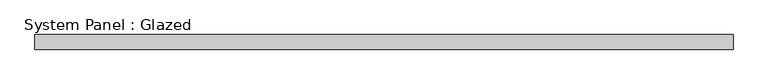
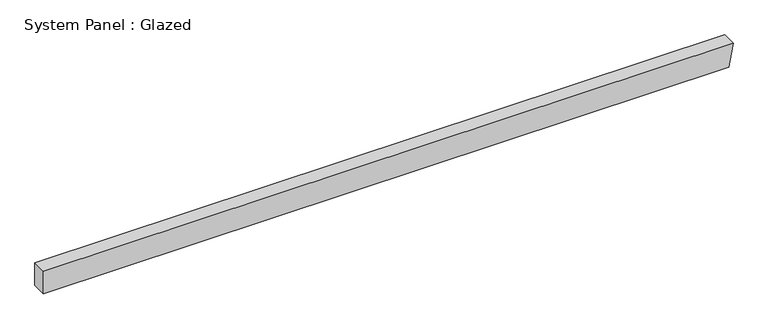
"""IFC4 building model written with IfcOpenShell, lengths in millimetres: plate geometry, System Panel : Glazed."""

from ifc_helpers import new_model, si_unit, frame, origin, place, context, project, spatial, polyline, outline, extrude, source, transform, mapped, element, save


def system_panel_glazed_abe217f1(model_context):
    return source(origin(), model_context, "Body", "SweptSolid", [
        extrude(outline(polyline([(0.0, -605.3523878), (0.0, 597.989887), (41.9143134, 605.3523878), (41.9143134, -605.3523878), (0.0, -605.3523878)])), frame((0.0, -44.45, 0.0), z_axis=(0.0, 1.0, 0.0), x_axis=(0.0, 0.0, 1.0)), (0.0, 0.0, 1.0), 25.4),
    ])


if __name__ == "__main__":
    model = new_model("IFC4")
    model_context = context("Model", 3, world=origin())
    ifc_project = project(units=[si_unit("LENGTHUNIT", "METRE", prefix="MILLI")], contexts=[model_context])
    site = spatial("IfcSite", under=ifc_project)
    building = spatial("IfcBuilding", under=site)
    placement = place(None, origin())
    system_panel_glazed_shape = system_panel_glazed_abe217f1(model_context)
    element("IfcPlate", 1, ObjectType="System Panel : Glazed", at=placement, inside=building, context=model_context, shape_type="MappedRepresentation", body=[
        mapped(system_panel_glazed_shape, transform((0.0, 0.0, 0.0), x_axis=(1.0, 0.0, 0.0), y_axis=(0.0, 1.0, 0.0), z_axis=(0.0, 0.0, 1.0))),
    ])
    save(model, "model.ifc")

# Revit data of these elements
# Type "System Panel : Glazed"
#   Construction Type Id = "GSP4R"
#   Analytic Construction = "1/8 in Pilkington single glazing"
#   Visual Light Transmittance = 0.9
#   Solar Heat Gain Coefficient = 0.86
#   Heat Transfer Coefficient (U) = 1.18115 BTU/(h·ft²·°F)
#   Define Thermal Properties by = 1
# Element 1 (IfcPlate, "System Panel : Glazed")
#   Materials on its faces: "Glass"
# Materials
#   "Glass": class "Glass", colour RGB 0 128 192, transparency 0.75, Description = "Soda Lime Glass", Cost = 0
